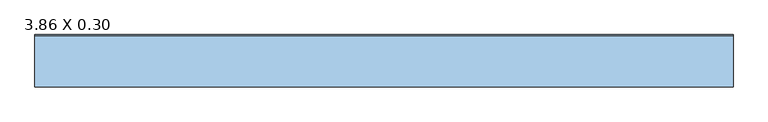
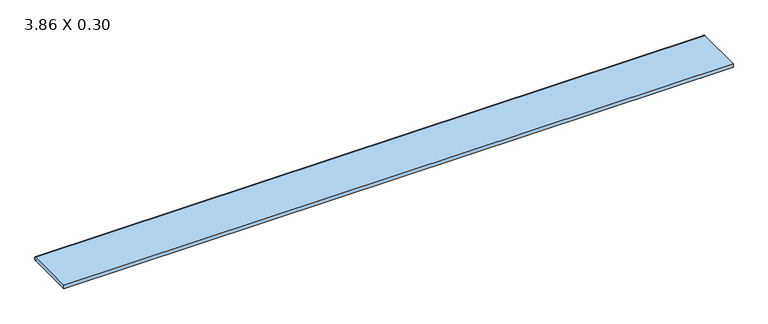
"""IFC4 building model written with IfcOpenShell, lengths in millimetres: window geometry, .CC_ND 300_PEDRA_PEITORIL RETO : 3.86 X 0.30."""

from ifc_helpers import new_model, si_unit, point, frame, frame_2d, origin, place, context, project, spatial, polyline, circle_curve, trimmed, segment, composite_curve, outline, extrude, source, transform, mapped, element, save


def window_3_86_x_0_30_427cbaa1(model_context):
    return source(origin(), model_context, "Body", "SweptSolid", [
        extrude(outline(composite_curve([segment(polyline([(144.4083081, 1480.0), (-129.9, 1480.0), (-129.9, 1500.0), (153.2808343, 1500.0)]), True, "CONTINUOUS"), segment(trimmed(circle_curve(frame_2d((153.2808343, 1493.3808343)), 6.6191657), [point((153.2808343, 1500.0))], [point((159.9, 1493.3808343))], False, "CARTESIAN"), True, "CONTINUOUS"), segment(polyline([(159.9, 1493.3808343), (159.9, 1480.0), (149.1619526, 1480.0), (149.1619526, 1488.1993124), (144.4083081, 1488.1993124), (144.4083081, 1480.0)]), True, "CONTINUOUS")], self_intersect=False)), frame((-1930.0, 0.0, 0.0), z_axis=(1.0, 0.0, 0.0), x_axis=(0.0, 1.0, 0.0)), (0.0, 0.0, 1.0), 3860.0),
    ])


if __name__ == "__main__":
    model = new_model("IFC4")
    model_context = context("Model", 3, world=origin())
    ifc_project = project(units=[si_unit("LENGTHUNIT", "METRE", prefix="MILLI")], contexts=[model_context])
    site = spatial("IfcSite", under=ifc_project)
    building = spatial("IfcBuilding", under=site)
    placement = place(None, origin())
    window_3_86_x_0_30_shape = window_3_86_x_0_30_427cbaa1(model_context)
    element("IfcWindow", 1, ObjectType=".CC_ND 300_PEDRA_PEITORIL RETO : 3.86 X 0.30", at=placement, inside=building, context=model_context, shape_type="MappedRepresentation", body=[
        mapped(window_3_86_x_0_30_shape, transform((0.0, 0.0, 0.0), x_axis=(1.0, 0.0, 0.0), y_axis=(0.0, 1.0, 0.0), z_axis=(0.0, 0.0, 1.0))),
    ])
    save(model, "model.ifc")

# Revit data of these elements
# Type ".CC_ND 300_PEDRA_PEITORIL RETO : 3.86 X 0.30"
#   Type Mark = "71"
#   Largura da pedra [instance default] = 0.26 m
#   Extensão interior peitoril [instance default] = 0.03 m
#   Extensão exterior peitoril [instance default] = 0.03 m
#   Espessura = 0.02 m
#   Comprimento = 3.86 m
#   Altura-padrão do peitoril = 1.48 m
#   Peitoril = .GRANITO_BRANCO_ITAUNAS
#   Rough Width = 0
#   Rough Height = 0
#   Height = 0
#   Wall Closure = (empty or 0)
#   Width = 0
# Element 1 (IfcWindow, ".CC_ND 300_PEDRA_PEITORIL RETO : 3.86 X 0.30")
#   Largura da pedra = 0.2898 m
#   Extensão interior peitoril = 0.00 m
#   Materials on its faces: ".GRANITO_BRANCO_ITAUNAS"
# Materials
#   ".GRANITO_BRANCO_ITAUNAS": class ".CC_PEDRA REVEST.", colour RGB 202 195 174, transparency 0, Description = "Revestimento em granito", Cost = 0
